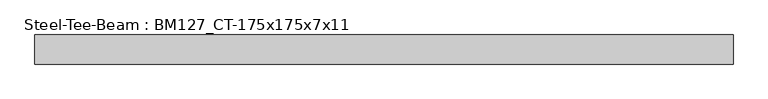
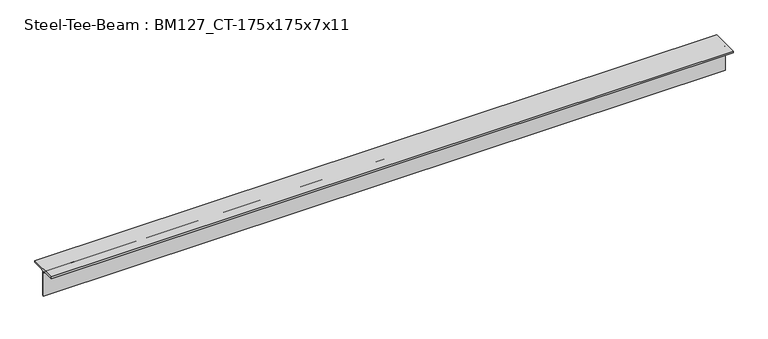
"""IFC4 building model written with IfcOpenShell, lengths in millimetres: beam geometry, Steel-Tee-Beam : BM127_CT-175x175x7x11."""

from ifc_helpers import new_model, si_unit, point, frame, frame_2d, origin, place, context, project, spatial, polyline, circle_curve, trimmed, segment, composite_curve, outline, extrude, source, transform, mapped, element, save


def steel_tee_beam_bm127_ct_175x175x7x11_e8e1f4b2(model_context):
    return source(origin(), model_context, "Body", "SweptSolid", [
        extrude(outline(composite_curve([segment(polyline([(-87.5, 87.5), (87.5, 87.5), (87.5, 76.5), (17.5, 76.5)]), True, "CONTINUOUS"), segment(trimmed(circle_curve(frame_2d((17.5, 62.5)), 14.0), [point((17.5, 76.5))], [point((3.5, 62.5))], True, "CARTESIAN"), True, "CONTINUOUS"), segment(polyline([(3.5, 62.5), (3.5, -87.5), (-3.5, -87.5), (-3.5, 62.5)]), True, "CONTINUOUS"), segment(trimmed(circle_curve(frame_2d((-17.5, 62.5)), 14.0), [point((-3.5, 62.5))], [point((-17.5, 76.5))], True, "CARTESIAN"), True, "CONTINUOUS"), segment(polyline([(-17.5, 76.5), (-87.5, 76.5), (-87.5, 87.5)]), True, "CONTINUOUS")], self_intersect=False)), frame((-1998.4928423, 0.0, 0.0), z_axis=(1.0, 0.0, 0.0), x_axis=(0.0, 1.0, 0.0)), (0.0, 0.0, 1.0), 4194.118334),
    ])


if __name__ == "__main__":
    model = new_model("IFC4")
    model_context = context("Model", 3, world=origin())
    ifc_project = project(units=[si_unit("LENGTHUNIT", "METRE", prefix="MILLI")], contexts=[model_context])
    site = spatial("IfcSite", under=ifc_project)
    building = spatial("IfcBuilding", under=site)
    placement = place(None, origin())
    steel_tee_beam_bm127_ct_175x175x7x11_shape = steel_tee_beam_bm127_ct_175x175x7x11_e8e1f4b2(model_context)
    element("IfcBeam", 1, ObjectType="Steel-Tee-Beam : BM127_CT-175x175x7x11", at=placement, inside=building, context=model_context, shape_type="MappedRepresentation", body=[
        mapped(steel_tee_beam_bm127_ct_175x175x7x11_shape, transform((0.0, 0.0, 0.0), x_axis=(1.0, 0.0, 0.0), y_axis=(0.0, 1.0, 0.0), z_axis=(0.0, 0.0, 1.0))),
    ])
    save(model, "model.ifc")

# Revit data of these elements
# Type "Steel-Tee-Beam : BM127_CT-175x175x7x11"
#   Surface Area = 0.00 m²/m
#   Section Area = 31.57 cm²
#   Mass per Unit Length = 24.80 kg/m
#   Length [instance default] = 1524 mm
#   bf = 175 mm
#   d = 175 mm
#   k = 25 mm
#   kr = 14 mm
#   tf = 11 mm
#   tw = 7 mm
#   hec_material4 [instance default] = none
#   hec_material3 [instance default] = none
#   hec_material2 [instance default] = none
#   hec_material1 [instance default] = none
#   Structural Material [instance default] = Steel, 45-345
#   Assembly Code = ""
# Element 1 (IfcBeam, "Steel-Tee-Beam : BM127_CT-175x175x7x11")
#   hec_material3 = F01AC000-00002_Building/Shelter Fire Proofing Work_Intumescent Coating Type_1 hr. rating (UL 1709))
#   hec_material2 = S01AA010-00002_Main Steel Structure Fabrication Work_Shelter/Building_Steel Painting/Coating_for Fireproofed Steel Surface, Surface Preparation & Primer Coat
#   hec_material1 = S03AA029-00001_Main Steel Structure Erection Work_Shelter/Building_Light Steel
#   Structural Material = S01AA003-00001_Main Steel Structure Fabrication Work_Shelter/Building_Light Steel - Standard
#   Materials on its faces: "S01AA003-00001_Main Steel Structure Fabrication Work_Shelter/Building_Light Steel - Standard"
# Materials
#   "Steel, 45-345": class "Metal", colour RGB 189 187 185, transparency 0, Description = "Steel 345 MPa", Cost = 0
#   "S01AA003-00001_Main Steel Structure Fabrication Work_Shelter/Building_Light Steel - Standard": class "Metal", colour RGB 120 120 120, transparency 0, Comments = "(30KG/M>Weight)", Description = "Structural steel 50ksi", W00) Work Master Code = "S01AA003-00001", W01) Work Master_Lv1 = "Main Steel Structure Fabrication Work", W02) Work Master_Lv2 = "Shelter/Building", W03) Work Master_Spec.1 = "Light Steel - Standard (30KG/M>Weight)", Cost = 0
#   "F01AC000-00002_Building/Shelter Fire Proofing Work_Intumescent Coating Type_1 hr. rating (UL 1709))": class "Metal", colour RGB 255 128 128, transparency 0, Description = "Paint finished steel", W00) Work Master Code = "F01AC000-00002", W01) Work Master_Lv1 = "Building/Shelter Fire Proofing Work", W02) Work Master_Lv2 = "Intumescent Coating Type", W03) Work Master_Spec.1 = "1 hr. rating (UL 1709)", Cost = 0
#   "S01AA010-00002_Main Steel Structure Fabrication Work_Shelter/Building_Steel Painting/Coating_for Fireproofed Steel Surface, Surface Preparation & Primer Coat": class "Metal", colour RGB 120 120 120, transparency 0, Description = "Paint finished steel", W00) Work Master Code = "SS01AA010-00002", W01) Work Master_Lv1 = "Main Steel Structure Fabrication Work", W02) Work Master_Lv2 = "Shelter/Building", W03) Work Master_Spec.1 = "Steel Painting/Coating", W04) Work Master_Spec.2 = "for Fireproofed Steel Surface, Surface Preparation & Primer Coat", Cost = 0
#   "S03AA029-00001_Main Steel Structure Erection Work_Shelter/Building_Light Steel": class "Metal", colour RGB 120 120 120, transparency 0, Comments = "(30KG/M>Weight)", Description = "Structural steel 50ksi", W00) Work Master Code = "S03AA029-00001", W01) Work Master_Lv1 = "Main Steel Structure Erection Work", W02) Work Master_Lv2 = "Shelter/Building", W03) Work Master_Spec.1 = "Light Steel (30KG/M>Weight)", Cost = 0
